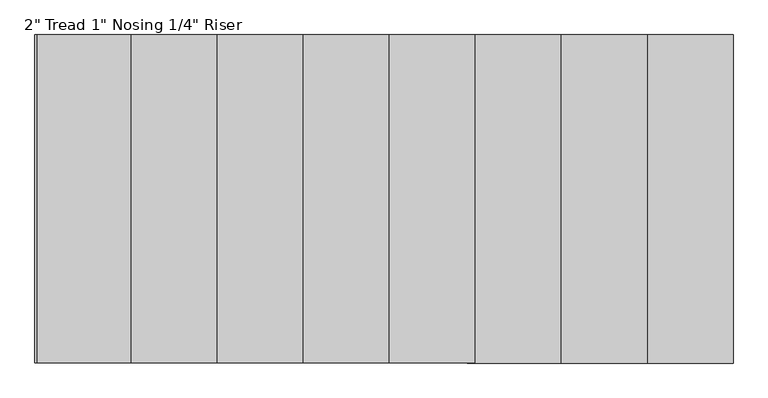
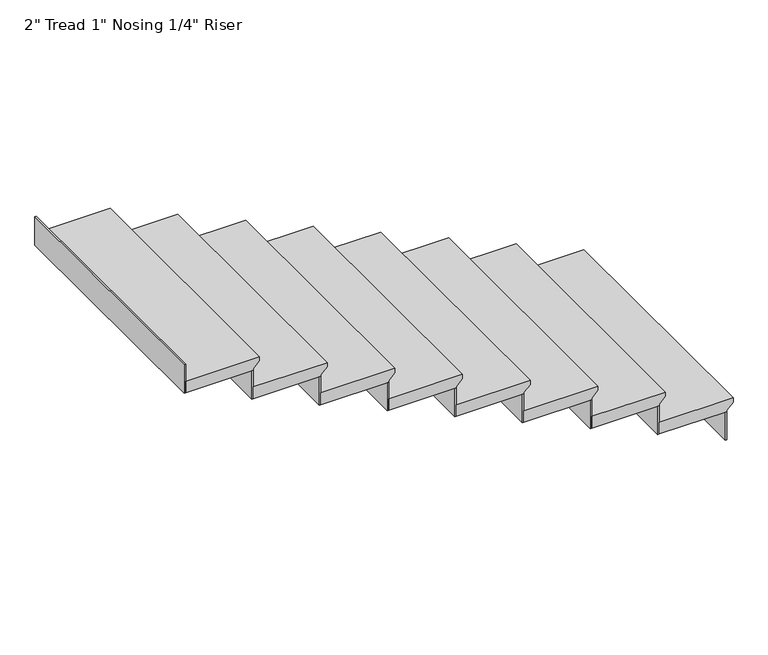
"""IFC4 building model written with IfcOpenShell, lengths in millimetres: stair flight geometry."""

from ifc_helpers import new_model, si_unit, origin, place, context, project, spatial, faceted_brep, source, transform, mapped, element, save


def stair_flight_a08092b1(model_context):
    return source(origin(), model_context, "Body", "Brep", [
        faceted_brep([(665956.388677, -549416.0413841, 1216.6256757), (665956.388677, -549416.0413841, 1235.6756757), (665956.388677, -550482.8413841, 1235.6756757), (665956.388677, -550482.8413841, 1216.6256757), (665930.988677, -549416.0413841, 1191.2256757), (665930.988677, -550482.8413841, 1191.2256757), (665651.588677, -549416.0413841, 1235.6756757), (665651.588677, -550482.8413841, 1235.6756757), (665930.988677, -550482.8413841, 1184.8756757), (665651.588677, -550482.8413841, 1184.8756757), (665651.588677, -549416.0413841, 1184.8756757), (665930.988677, -549416.0413841, 1184.8756757)], [[[0, 1, 2, 3]], [[4, 0, 3, 5]], [[2, 1, 6, 7]], [[8, 9, 10, 11]], [[2, 7, 9, 8, 5, 3]], [[8, 11, 4, 5]], [[6, 1, 0, 4, 11, 10]], [[7, 6, 10, 9]]]),
        faceted_brep([(665930.988677, -549416.0413841, 1184.8756757), (665930.988677, -549416.0413841, 1061.3081081), (665924.638677, -549416.0413841, 1061.3081081), (665924.638677, -549416.0413841, 1184.8756757), (665930.988677, -550482.8413841, 1184.8756757), (665924.638677, -550482.8413841, 1184.8756757), (665924.638677, -550482.8413841, 1061.3081081), (665930.988677, -550482.8413841, 1061.3081081)], [[[0, 1, 2, 3]], [[4, 5, 6, 7]], [[1, 0, 4, 7]], [[2, 1, 7, 6]], [[3, 2, 6, 5]], [[0, 3, 5, 4]]]),
        faceted_brep([(665651.588677, -549416.0413841, 1308.4432432), (665651.588677, -549416.0413841, 1184.8756757), (665645.238677, -549416.0413841, 1184.8756757), (665645.238677, -549416.0413841, 1308.4432432), (665651.588677, -550482.8413841, 1308.4432432), (665645.238677, -550482.8413841, 1308.4432432), (665645.238677, -550482.8413841, 1184.8756757), (665651.588677, -550482.8413841, 1184.8756757)], [[[0, 1, 2, 3]], [[4, 5, 6, 7]], [[1, 0, 4, 7]], [[2, 1, 7, 6]], [[3, 2, 6, 5]], [[0, 3, 5, 4]]]),
        faceted_brep([(665676.988677, -550482.8413841, 1359.2432432), (665676.988677, -549416.0413841, 1359.2432432), (665372.188677, -549416.0413841, 1359.2432432), (665372.188677, -550482.8413841, 1359.2432432), (665651.588677, -550482.8413841, 1308.4432432), (665372.188677, -550482.8413841, 1308.4432432), (665372.188677, -549416.0413841, 1308.4432432), (665651.588677, -549416.0413841, 1308.4432432), (665651.588677, -550482.8413841, 1314.7932432), (665676.988677, -550482.8413841, 1340.1932432), (665651.588677, -549416.0413841, 1314.7932432), (665676.988677, -549416.0413841, 1340.1932432)], [[[0, 1, 2, 3]], [[4, 5, 6, 7]], [[0, 3, 5, 4, 8, 9]], [[4, 7, 10, 8]], [[2, 1, 11, 10, 7, 6]], [[3, 2, 6, 5]], [[11, 1, 0, 9]], [[10, 11, 9, 8]]]),
        faceted_brep([(665372.188677, -549416.0413841, 1432.0108108), (665372.188677, -549416.0413841, 1308.4432432), (665365.838677, -549416.0413841, 1308.4432432), (665365.838677, -549416.0413841, 1432.0108108), (665372.188677, -550482.8413841, 1432.0108108), (665365.838677, -550482.8413841, 1432.0108108), (665365.838677, -550482.8413841, 1308.4432432), (665372.188677, -550482.8413841, 1308.4432432)], [[[0, 1, 2, 3]], [[4, 5, 6, 7]], [[1, 0, 4, 7]], [[2, 1, 7, 6]], [[3, 2, 6, 5]], [[0, 3, 5, 4]]]),
        faceted_brep([(665397.588677, -550482.8413841, 1482.8108108), (665397.588677, -549416.0413841, 1482.8108108), (665092.788677, -549416.0413841, 1482.8108108), (665092.788677, -550482.8413841, 1482.8108108), (665372.188677, -550482.8413841, 1432.0108108), (665092.788677, -550482.8413841, 1432.0108108), (665092.788677, -549416.0413841, 1432.0108108), (665372.188677, -549416.0413841, 1432.0108108), (665372.188677, -550482.8413841, 1438.3608108), (665397.588677, -550482.8413841, 1463.7608108), (665372.188677, -549416.0413841, 1438.3608108), (665397.588677, -549416.0413841, 1463.7608108)], [[[0, 1, 2, 3]], [[4, 5, 6, 7]], [[0, 3, 5, 4, 8, 9]], [[4, 7, 10, 8]], [[2, 1, 11, 10, 7, 6]], [[3, 2, 6, 5]], [[11, 1, 0, 9]], [[10, 11, 9, 8]]]),
        faceted_brep([(665092.788677, -549416.0413841, 1555.5783784), (665092.788677, -549416.0413841, 1432.0108108), (665086.438677, -549416.0413841, 1432.0108108), (665086.438677, -549416.0413841, 1555.5783784), (665092.788677, -550482.8413841, 1555.5783784), (665086.438677, -550482.8413841, 1555.5783784), (665086.438677, -550482.8413841, 1432.0108108), (665092.788677, -550482.8413841, 1432.0108108)], [[[0, 1, 2, 3]], [[4, 5, 6, 7]], [[1, 0, 4, 7]], [[2, 1, 7, 6]], [[3, 2, 6, 5]], [[0, 3, 5, 4]]]),
        faceted_brep([(665118.188677, -550482.8413841, 1606.3783784), (665118.188677, -549416.0413841, 1606.3783784), (664813.388677, -549416.0413841, 1606.3783784), (664813.388677, -550482.8413841, 1606.3783784), (665092.788677, -550482.8413841, 1555.5783784), (664813.388677, -550482.8413841, 1555.5783784), (664813.388677, -549416.0413841, 1555.5783784), (665092.788677, -549416.0413841, 1555.5783784), (665092.788677, -550482.8413841, 1561.9283784), (665118.188677, -550482.8413841, 1587.3283784), (665092.788677, -549416.0413841, 1561.9283784), (665118.188677, -549416.0413841, 1587.3283784)], [[[0, 1, 2, 3]], [[4, 5, 6, 7]], [[0, 3, 5, 4, 8, 9]], [[4, 7, 10, 8]], [[2, 1, 11, 10, 7, 6]], [[3, 2, 6, 5]], [[11, 1, 0, 9]], [[10, 11, 9, 8]]]),
        faceted_brep([(664813.388677, -549416.0413841, 1679.1459459), (664813.388677, -549416.0413841, 1555.5783784), (664807.038677, -549416.0413841, 1555.5783784), (664807.038677, -549416.0413841, 1679.1459459), (664813.388677, -550482.8413841, 1679.1459459), (664807.038677, -550482.8413841, 1679.1459459), (664807.038677, -550482.8413841, 1555.5783784), (664813.388677, -550482.8413841, 1555.5783784)], [[[0, 1, 2, 3]], [[4, 5, 6, 7]], [[1, 0, 4, 7]], [[2, 1, 7, 6]], [[3, 2, 6, 5]], [[0, 3, 5, 4]]]),
        faceted_brep([(664838.788677, -550482.8413841, 1729.9459459), (664838.788677, -549416.0413841, 1729.9459459), (664533.988677, -549416.0413841, 1729.9459459), (664533.988677, -550482.8413841, 1729.9459459), (664813.388677, -550482.8413841, 1679.1459459), (664533.988677, -550482.8413841, 1679.1459459), (664533.988677, -549416.0413841, 1679.1459459), (664813.388677, -549416.0413841, 1679.1459459), (664813.388677, -550482.8413841, 1685.4959459), (664838.788677, -550482.8413841, 1710.8959459), (664813.388677, -549416.0413841, 1685.4959459), (664838.788677, -549416.0413841, 1710.8959459)], [[[0, 1, 2, 3]], [[4, 5, 6, 7]], [[0, 3, 5, 4, 8, 9]], [[4, 7, 10, 8]], [[2, 1, 11, 10, 7, 6]], [[3, 2, 6, 5]], [[11, 1, 0, 9]], [[10, 11, 9, 8]]]),
        faceted_brep([(664533.988677, -549416.0413841, 1802.7135135), (664533.988677, -549416.0413841, 1679.1459459), (664527.638677, -549416.0413841, 1679.1459459), (664527.638677, -549416.0413841, 1802.7135135), (664533.988677, -550482.8413841, 1802.7135135), (664527.638677, -550482.8413841, 1802.7135135), (664527.638677, -550482.8413841, 1679.1459459), (664533.988677, -550482.8413841, 1679.1459459)], [[[0, 1, 2, 3]], [[4, 5, 6, 7]], [[1, 0, 4, 7]], [[2, 1, 7, 6]], [[3, 2, 6, 5]], [[0, 3, 5, 4]]]),
        faceted_brep([(664559.388677, -550482.8413841, 1853.5135135), (664559.388677, -549416.0413841, 1853.5135135), (664254.588677, -549416.0413841, 1853.5135135), (664254.588677, -550482.8413841, 1853.5135135), (664533.988677, -550482.8413841, 1802.7135135), (664254.588677, -550482.8413841, 1802.7135135), (664254.588677, -549416.0413841, 1802.7135135), (664533.988677, -549416.0413841, 1802.7135135), (664533.988677, -550482.8413841, 1809.0635135), (664559.388677, -550482.8413841, 1834.4635135), (664533.988677, -549416.0413841, 1809.0635135), (664559.388677, -549416.0413841, 1834.4635135)], [[[0, 1, 2, 3]], [[4, 5, 6, 7]], [[0, 3, 5, 4, 8, 9]], [[4, 7, 10, 8]], [[2, 1, 11, 10, 7, 6]], [[3, 2, 6, 5]], [[11, 1, 0, 9]], [[10, 11, 9, 8]]]),
        faceted_brep([(664254.588677, -549416.0413841, 1926.2810811), (664254.588677, -549416.0413841, 1802.7135135), (664248.238677, -549416.0413841, 1802.7135135), (664248.238677, -549416.0413841, 1926.2810811), (664254.588677, -550482.8413841, 1926.2810811), (664248.238677, -550482.8413841, 1926.2810811), (664248.238677, -550482.8413841, 1802.7135135), (664254.588677, -550482.8413841, 1802.7135135)], [[[0, 1, 2, 3]], [[4, 5, 6, 7]], [[1, 0, 4, 7]], [[2, 1, 7, 6]], [[3, 2, 6, 5]], [[0, 3, 5, 4]]]),
        faceted_brep([(664279.988677, -550482.8413841, 1977.0810811), (664279.988677, -549416.0413841, 1977.0810811), (663975.188677, -549416.0413841, 1977.0810811), (663975.188677, -550482.8413841, 1977.0810811), (664254.588677, -550482.8413841, 1926.2810811), (663975.188677, -550482.8413841, 1926.2810811), (663975.188677, -549416.0413841, 1926.2810811), (664254.588677, -549416.0413841, 1926.2810811), (664254.588677, -550482.8413841, 1932.6310811), (664279.988677, -550482.8413841, 1958.0310811), (664254.588677, -549416.0413841, 1932.6310811), (664279.988677, -549416.0413841, 1958.0310811)], [[[0, 1, 2, 3]], [[4, 5, 6, 7]], [[0, 3, 5, 4, 8, 9]], [[4, 7, 10, 8]], [[2, 1, 11, 10, 7, 6]], [[3, 2, 6, 5]], [[11, 1, 0, 9]], [[10, 11, 9, 8]]]),
        faceted_brep([(663695.788677, -549416.0413841, 2173.4162162), (663695.788677, -549416.0413841, 2049.8486486), (663689.438677, -549416.0413841, 2049.8486486), (663689.438677, -549416.0413841, 2173.4162162), (663695.788677, -550482.8413841, 2173.4162162), (663689.438677, -550482.8413841, 2173.4162162), (663689.438677, -550482.8413841, 2049.8486486), (663695.788677, -550482.8413841, 2049.8486486)], [[[0, 1, 2, 3]], [[4, 5, 6, 7]], [[1, 0, 4, 7]], [[2, 1, 7, 6]], [[3, 2, 6, 5]], [[0, 3, 5, 4]]]),
        faceted_brep([(663975.188677, -549416.0413841, 2049.8486486), (663975.188677, -549416.0413841, 1926.2810811), (663968.838677, -549416.0413841, 1926.2810811), (663968.838677, -549416.0413841, 2049.8486486), (663975.188677, -550482.8413841, 2049.8486486), (663968.838677, -550482.8413841, 2049.8486486), (663968.838677, -550482.8413841, 1926.2810811), (663975.188677, -550482.8413841, 1926.2810811)], [[[0, 1, 2, 3]], [[4, 5, 6, 7]], [[1, 0, 4, 7]], [[2, 1, 7, 6]], [[3, 2, 6, 5]], [[0, 3, 5, 4]]]),
        faceted_brep([(664000.588677, -550482.8413841, 2100.6486486), (664000.588677, -549416.0413841, 2100.6486486), (663721.188677, -549416.0413841, 2100.6486486), (663695.788677, -549416.0413841, 2100.6486486), (663695.788677, -550482.8413841, 2100.6486486), (663975.188677, -550482.8413841, 2049.8486486), (663695.788677, -550482.8413841, 2049.8486486), (663695.788677, -549416.0413841, 2049.8486486), (663721.188677, -549416.0413841, 2049.8486486), (663975.188677, -549416.0413841, 2049.8486486), (663975.188677, -550482.8413841, 2056.1986486), (664000.588677, -550482.8413841, 2081.5986486), (663975.188677, -549416.0413841, 2056.1986486), (664000.588677, -549416.0413841, 2081.5986486)], [[[0, 1, 2, 3, 4]], [[5, 6, 7, 8, 9]], [[0, 4, 6, 5, 10, 11]], [[5, 9, 12, 10]], [[2, 1, 13, 12, 9, 8]], [[3, 2, 8, 7]], [[4, 3, 7, 6]], [[13, 1, 0, 11]], [[12, 13, 11, 10]]]),
    ])


if __name__ == "__main__":
    model = new_model("IFC4")
    model_context = context("Model", 3, world=origin())
    ifc_project = project(units=[si_unit("LENGTHUNIT", "METRE", prefix="MILLI")], contexts=[model_context])
    site = spatial("IfcSite", under=ifc_project)
    building = spatial("IfcBuilding", under=site)
    placement = place(None, origin())
    stair_flight_shape = stair_flight_a08092b1(model_context)
    element("IfcStairFlight", 1, ObjectType="2\" Tread 1\" Nosing 1/4\" Riser", at=placement, inside=building, context=model_context, shape_type="MappedRepresentation", body=[
        mapped(stair_flight_shape, transform((0.0, 0.0, 0.0), x_axis=(1.0, 0.0, 0.0), y_axis=(0.0, 1.0, 0.0), z_axis=(0.0, 0.0, 1.0))),
    ])
    save(model, "model.ifc")
